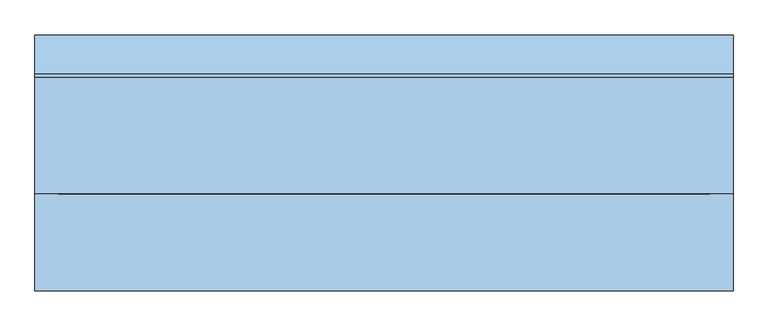
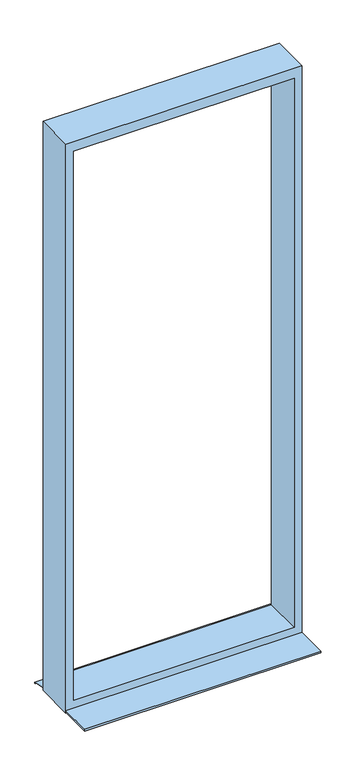
"""IFC4 building model written with IfcOpenShell, lengths in millimetres: window geometry, Fenster - Festverglasung : Feste Verglasung 4.58 x 1.8."""

from ifc_helpers import new_model, si_unit, frame, origin, place, context, project, spatial, polyline, outline, extrude, source, transform, mapped, element, save


def window_cdc7c389(model_context):
    return source(origin(), model_context, "Body", "SweptSolid", [
        extrude(outline(polyline([(5580.0, 900.0), (5580.0, -900.0), (1000.0, -900.0), (1000.0, 900.0), (5580.0, 900.0)]), holes=[polyline([(5500.0, 840.0), (1080.0, 840.0), (1080.0, -840.0), (5500.0, -840.0), (5500.0, 840.0)])]), frame((0.0, -80.0, 0.0), z_axis=(0.0, 1.0, 0.0), x_axis=(0.0, 0.0, 1.0)), (0.0, 0.0, 1.0), 300.0),
        extrude(outline(polyline([(-900.0, -330.0), (-900.0, -80.0), (900.0, -80.0), (900.0, -330.0), (-900.0, -330.0)])), frame((0.0, 0.0, 1005.0), z_axis=(0.0, 0.0, 1.0), x_axis=(1.0, 0.0, 0.0)), (0.0, 0.0, 1.0), 15.0),
        extrude(outline(polyline([(230.0221543, 1020.0), (330.0, 1000.0), (330.0, 990.0), (328.0, 990.0), (328.0, 998.3604634), (229.8240723, 1018.0), (220.0, 1018.0), (220.0, 1020.0), (230.0221543, 1020.0)])), frame((-900.0, 0.0, 0.0), z_axis=(1.0, 0.0, 0.0), x_axis=(0.0, 1.0, 0.0)), (0.0, 0.0, 1.0), 1800.0),
    ])


if __name__ == "__main__":
    model = new_model("IFC4")
    model_context = context("Model", 3, world=origin())
    ifc_project = project(units=[si_unit("LENGTHUNIT", "METRE", prefix="MILLI")], contexts=[model_context])
    site = spatial("IfcSite", under=ifc_project)
    building = spatial("IfcBuilding", under=site)
    placement = place(None, origin())
    window_shape = window_cdc7c389(model_context)
    element("IfcWindow", 1, ObjectType="Fenster - Festverglasung : Feste Verglasung 4.58 x 1.8", at=placement, inside=building, context=model_context, shape_type="MappedRepresentation", body=[
        mapped(window_shape, transform((0.0, 0.0, 0.0), x_axis=(1.0, 0.0, 0.0), y_axis=(0.0, 1.0, 0.0), z_axis=(0.0, 0.0, 1.0))),
    ])
    save(model, "model.ifc")

# Revit data of these elements
# Type "Fenster - Festverglasung : Feste Verglasung 4.58 x 1.8"
#   Type Mark = "52"
#   Operation = "SinglePanel"
#   Keynote = "16.05.01"
#   Visual Light Transmittance = 0.9
#   Solar Heat Gain Coefficient = 0.78
#   Rough Width = 1.800 m
#   Rough Height = 4.580 m
#   Heat Transfer Coefficient (U) = 3.6886 W/(m²·K)
#   Rahmentiefe = 0.300 m
#   Rahmenhöhe unten = 0.080 m
#   Höhe oberer  Rahmen = 0.080 m
#   Rahmenbreite = 0.060 m
#   Height = 4.580 m
#   Einbautiefe (von außen) [instance default] = 0.080 m
#   Width = 1.800 m
#   Wall Closure = 3
#   Bild [instance default] = none
#   Glas [instance default] = none
#   Innere Fensterbank [instance default] = none
#   Äußere Fensterbank [instance default] = none
#   Construction Type Id = ""
#   Analytic Construction = (empty or 0)
# Element 1 (IfcWindow, "Fenster - Festverglasung : Feste Verglasung 4.58 x 1.8")
#   Materials on its faces: "Kunststoff - Weiß", "Holz - Birke"
# Materials
#   "Kunststoff - Weiß": class "Kunststoff", colour RGB 249 249 249, transparency 0, Cost = 0
#   "Holz - Birke": class "Holz", colour RGB 213 164 103, transparency 0, Cost = 0
